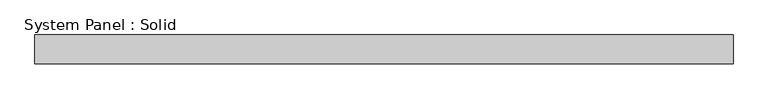
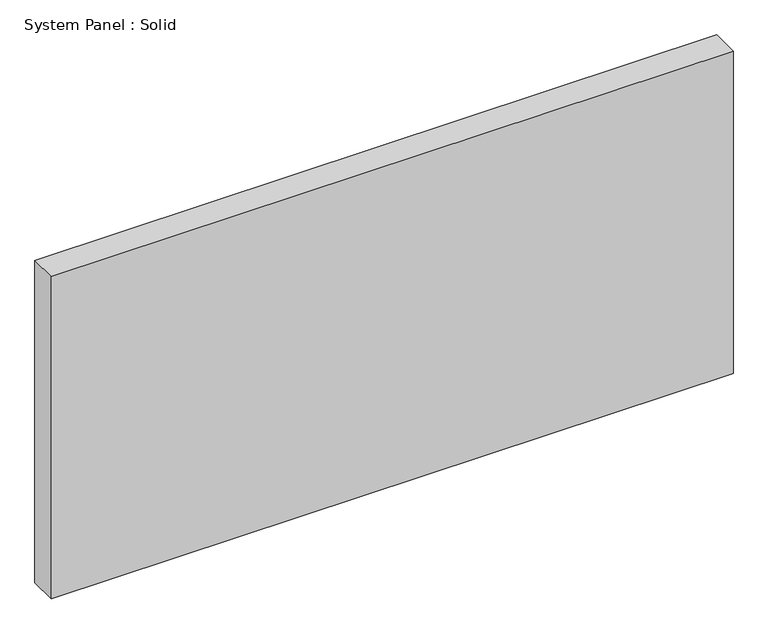
"""IFC4 building model written with IfcOpenShell, lengths in millimetres: plate geometry, System Panel : Solid."""

from ifc_helpers import new_model, si_unit, origin, origin_with_axes, place, context, project, spatial, polyline, outline, extrude, source, transform, mapped, element, save


def system_panel_solid_0358887a(model_context):
    return source(origin(), model_context, "Body", "SweptSolid", [
        extrude(outline(polyline([(724.9999999, -10.5), (-724.9999999, -10.5), (-724.9999999, 49.5), (724.9999999, 49.5), (724.9999999, -10.5)])), origin_with_axes(), (0.0, 0.0, 1.0), 725.0),
    ])


if __name__ == "__main__":
    model = new_model("IFC4")
    model_context = context("Model", 3, world=origin())
    ifc_project = project(units=[si_unit("LENGTHUNIT", "METRE", prefix="MILLI")], contexts=[model_context])
    site = spatial("IfcSite", under=ifc_project)
    building = spatial("IfcBuilding", under=site)
    placement = place(None, origin())
    system_panel_solid_shape = system_panel_solid_0358887a(model_context)
    element("IfcPlate", 1, ObjectType="System Panel : Solid", at=placement, inside=building, context=model_context, shape_type="MappedRepresentation", body=[
        mapped(system_panel_solid_shape, transform((0.0, 0.0, 0.0), x_axis=(1.0, 0.0, 0.0), y_axis=(0.0, 1.0, 0.0), z_axis=(0.0, 0.0, 1.0))),
    ])
    save(model, "model.ifc")

# Revit data of these elements
# Project information
#   Project Issue Date = "Issue Date"
#   Project Status = "Project Status"
#   Client Name = "Owner"
#   Project Address = "Enter address here"
#   Project Name = "Project Name"
#   Project Number = "Project Number"
# Type "System Panel : Solid"
#   Keynote = "H11"
#   Construction Type Id = "MDOOR"
#   Analytic Construction = "Metal"
#   Visual Light Transmittance = 0
#   Solar Heat Gain Coefficient = 0
#   Heat Transfer Coefficient (U) = 3.7021 W/(m²·K)
# Element 1 (IfcPlate, "System Panel : Solid")
#   Materials on its faces: "Default"
# Materials
#   "Default": class "Miscellaneous", colour RGB 127 127 127, transparency 0, Comments = "Rendering appearance not upgraded ", Cost = 0
